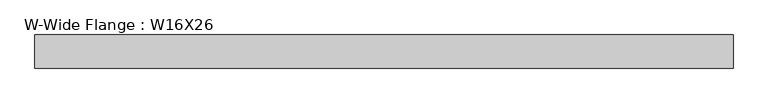
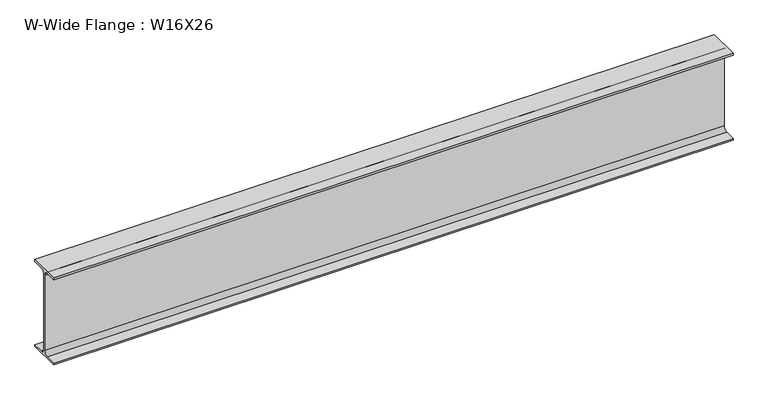
"""IFC4 building model written with IfcOpenShell, lengths in millimetres: beam geometry, W-Wide Flange : W16X26."""

from ifc_helpers import new_model, si_unit, point, frame, frame_2d, origin, place, context, project, spatial, polyline, circle_curve, trimmed, segment, composite_curve, outline, extrude, source, transform, mapped, element, save


def w_wide_flange_w16x26_f2db45cd(model_context):
    return source(origin(), model_context, "Body", "SweptSolid", [
        extrude(outline(composite_curve([segment(polyline([(69.85, -190.627), (69.85, -199.39), (-69.85, -199.39), (-69.85, -190.627), (-21.3995, -190.627)]), True, "CONTINUOUS"), segment(trimmed(circle_curve(frame_2d((-21.3995, -172.4025)), 18.2245), [point((-21.3995, -190.627))], [point((-3.175, -172.4025))], True, "CARTESIAN"), True, "CONTINUOUS"), segment(polyline([(-3.175, -172.4025), (-3.175, 172.4025)]), True, "CONTINUOUS"), segment(trimmed(circle_curve(frame_2d((-21.3995, 172.4025)), 18.2245), [point((-3.175, 172.4025))], [point((-21.3995, 190.627))], True, "CARTESIAN"), True, "CONTINUOUS"), segment(polyline([(-21.3995, 190.627), (-69.85, 190.627), (-69.85, 199.39), (69.85, 199.39), (69.85, 190.627), (21.3995, 190.627)]), True, "CONTINUOUS"), segment(trimmed(circle_curve(frame_2d((21.3995, 172.4025)), 18.2245), [point((21.3995, 190.627))], [point((3.175, 172.4025))], True, "CARTESIAN"), True, "CONTINUOUS"), segment(polyline([(3.175, 172.4025), (3.175, -172.4025)]), True, "CONTINUOUS"), segment(trimmed(circle_curve(frame_2d((21.3995, -172.4025)), 18.2245), [point((3.175, -172.4025))], [point((21.3995, -190.627))], True, "CARTESIAN"), True, "CONTINUOUS"), segment(polyline([(21.3995, -190.627), (69.85, -190.627)]), True, "CONTINUOUS")], self_intersect=False)), frame((-1472.438, 0.0, 0.0), z_axis=(1.0, 0.0, 0.0), x_axis=(0.0, 1.0, 0.0)), (0.0, 0.0, 1.0), 2945.638),
    ])


if __name__ == "__main__":
    model = new_model("IFC4")
    model_context = context("Model", 3, world=origin())
    ifc_project = project(units=[si_unit("LENGTHUNIT", "METRE", prefix="MILLI")], contexts=[model_context])
    site = spatial("IfcSite", under=ifc_project)
    building = spatial("IfcBuilding", under=site)
    placement = place(None, origin())
    w_wide_flange_w16x26_shape = w_wide_flange_w16x26_f2db45cd(model_context)
    element("IfcBeam", 1, ObjectType="W-Wide Flange : W16X26", at=placement, inside=building, context=model_context, shape_type="MappedRepresentation", body=[
        mapped(w_wide_flange_w16x26_shape, transform((0.0, 0.0, 0.0), x_axis=(1.0, 0.0, 0.0), y_axis=(0.0, 1.0, 0.0), z_axis=(0.0, 0.0, 1.0))),
    ])
    save(model, "model.ifc")

# Revit data of these elements
# Type "W-Wide Flange : W16X26"
#   Assembly Code = "B10"
#   W = 26
#   Length [instance default] = 5' - 0"
#   bf = 0' - 5 1/2"
#   d = 1' - 3.7"
#   k = 0' - 1 1/16"
#   k2 = 0' - 0.7175"
#   tf = 0' - 0.345"
#   tw = 0' - 0 1/4"
#   A = 0.0533333 SF
#   Structural Material [instance default] = Steel ASTM A992
# Element 1 (IfcBeam, "W-Wide Flange : W16X26")
#   Materials on its faces: "Steel ASTM A992"
# Materials
#   "Steel ASTM A992": class "Metal", colour RGB 199 199 199, transparency 0, Description = "Structural steel 50ksi", Cost = 0
